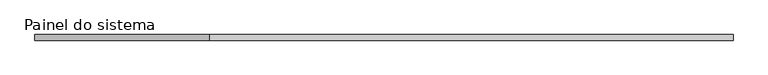
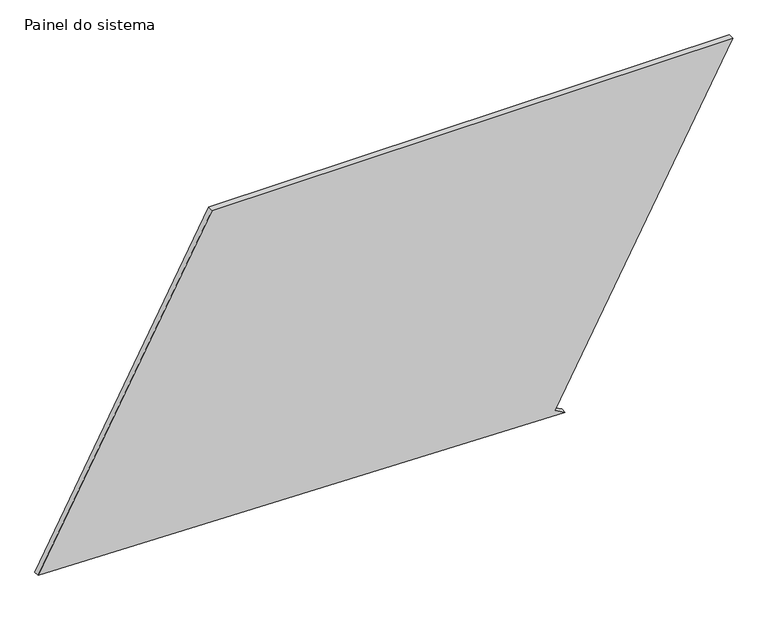
"""IFC4 building model written with IfcOpenShell, lengths in millimetres: plate geometry, Painel do sistema : Envidraçado."""

from ifc_helpers import new_model, si_unit, frame, origin, place, context, project, spatial, polyline, outline, extrude, source, transform, mapped, element, save


def painel_do_sistema_28591016(model_context):
    return source(origin(), model_context, "Body", "SweptSolid", [
        extrude(outline(polyline([(0.0, 806.5781037), (23.5917513, 762.493761), (1513.6028502, 1559.8737189), (1513.6028502, -778.6609729), (53.8023491, -1559.8737189), (0.0, 806.5781037)])), frame((0.0, 24.5, 0.0), z_axis=(0.0, 1.0, 0.0), x_axis=(0.0, 0.0, 1.0)), (0.0, 0.0, 1.0), 25.0),
    ])


if __name__ == "__main__":
    model = new_model("IFC4")
    model_context = context("Model", 3, world=origin())
    ifc_project = project(units=[si_unit("LENGTHUNIT", "METRE", prefix="MILLI")], contexts=[model_context])
    site = spatial("IfcSite", under=ifc_project)
    building = spatial("IfcBuilding", under=site)
    placement = place(None, origin())
    painel_do_sistema_shape = painel_do_sistema_28591016(model_context)
    element("IfcPlate", 1, ObjectType="Painel do sistema : Envidraçado", at=placement, inside=building, context=model_context, shape_type="MappedRepresentation", body=[
        mapped(painel_do_sistema_shape, transform((0.0, 0.0, 0.0), x_axis=(1.0, 0.0, 0.0), y_axis=(0.0, 1.0, 0.0), z_axis=(0.0, 0.0, 1.0))),
    ])
    save(model, "model.ifc")

# Revit data of these elements
# Type "Painel do sistema : Envidraçado"
#   Construction Type Id = "GSP4R"
#   Analytic Construction = "Vidraça única Pilkington 1/8 pol"
#   Visual Light Transmittance = 0.9
#   Solar Heat Gain Coefficient = 0.86
#   Heat Transfer Coefficient (U) = 6.7069 W/(m²·K)
# Element 1 (IfcPlate, "Painel do sistema : Envidraçado")
#   Materials on its faces: "Vidro"
# Materials
#   "Vidro": class "Vidro", colour RGB 0 128 192, transparency 0.9, Description = "Vidro de sílica", Cost = 0
